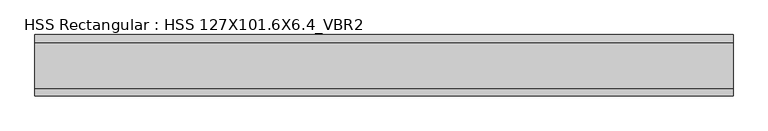
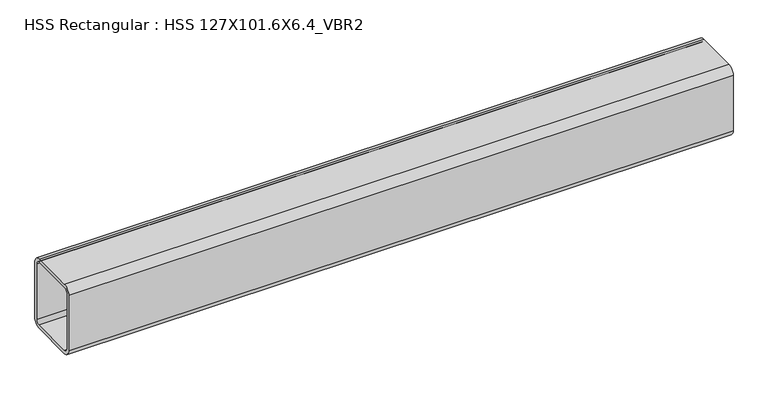
"""IFC4 building model written with IfcOpenShell, lengths in millimetres: member geometry, HSS Rectangular : HSS 127X101.6X6.4_VBR2."""

from ifc_helpers import new_model, si_unit, point, frame, frame_2d, origin, place, context, project, spatial, polyline, circle_curve, trimmed, segment, composite_curve, outline, extrude, source, transform, mapped, element, save


def hss_rectangular_hss_127x101_6x6_4_vbr2_0793e8e8(model_context):
    return source(origin(), model_context, "Body", "SweptSolid", [
        extrude(outline(composite_curve([segment(polyline([(50.8, 50.8), (50.8, -50.8)]), True, "CONTINUOUS"), segment(trimmed(circle_curve(frame_2d((38.1, -50.8)), 12.7), [point((50.8, -50.8))], [point((38.1, -63.5))], False, "CARTESIAN"), True, "CONTINUOUS"), segment(polyline([(38.1, -63.5), (-38.1, -63.5)]), True, "CONTINUOUS"), segment(trimmed(circle_curve(frame_2d((-38.1, -50.8)), 12.7), [point((-38.1, -63.5))], [point((-50.8, -50.8))], False, "CARTESIAN"), True, "CONTINUOUS"), segment(polyline([(-50.8, -50.8), (-50.8, 50.8)]), True, "CONTINUOUS"), segment(trimmed(circle_curve(frame_2d((-38.1, 50.8)), 12.7), [point((-50.8, 50.8))], [point((-38.1, 63.5))], False, "CARTESIAN"), True, "CONTINUOUS"), segment(polyline([(-38.1, 63.5), (38.1, 63.5)]), True, "CONTINUOUS"), segment(trimmed(circle_curve(frame_2d((38.1, 50.8)), 12.7), [point((38.1, 63.5))], [point((50.8, 50.8))], False, "CARTESIAN"), True, "CONTINUOUS")], self_intersect=False), holes=[composite_curve([segment(trimmed(circle_curve(frame_2d((-38.1, 50.8)), 6.35), [point((-38.1, 57.15))], [point((-44.45, 50.8))], True, "CARTESIAN"), True, "CONTINUOUS"), segment(polyline([(-44.45, 50.8), (-44.45, -50.8)]), True, "CONTINUOUS"), segment(trimmed(circle_curve(frame_2d((-38.1, -50.8)), 6.35), [point((-44.45, -50.8))], [point((-38.1, -57.15))], True, "CARTESIAN"), True, "CONTINUOUS"), segment(polyline([(-38.1, -57.15), (38.1, -57.15)]), True, "CONTINUOUS"), segment(trimmed(circle_curve(frame_2d((38.1, -50.8)), 6.35), [point((38.1, -57.15))], [point((44.45, -50.8))], True, "CARTESIAN"), True, "CONTINUOUS"), segment(polyline([(44.45, -50.8), (44.45, 50.8)]), True, "CONTINUOUS"), segment(trimmed(circle_curve(frame_2d((38.1, 50.8)), 6.35), [point((44.45, 50.8))], [point((38.1, 57.15))], True, "CARTESIAN"), True, "CONTINUOUS"), segment(polyline([(38.1, 57.15), (-38.1, 57.15)]), True, "CONTINUOUS")], self_intersect=False)]), frame((-613.1910365, 0.0, 0.0), z_axis=(1.0, 0.0, 0.0), x_axis=(0.0, 1.0, 0.0)), (0.0, 0.0, 1.0), 1153.1966521),
    ])


if __name__ == "__main__":
    model = new_model("IFC4")
    model_context = context("Model", 3, world=origin())
    ifc_project = project(units=[si_unit("LENGTHUNIT", "METRE", prefix="MILLI")], contexts=[model_context])
    site = spatial("IfcSite", under=ifc_project)
    building = spatial("IfcBuilding", under=site)
    placement = place(None, origin())
    hss_rectangular_hss_127x101_6x6_4_vbr2_shape = hss_rectangular_hss_127x101_6x6_4_vbr2_0793e8e8(model_context)
    element("IfcMember", 1, ObjectType="HSS Rectangular : HSS 127X101.6X6.4_VBR2", at=placement, inside=building, context=model_context, shape_type="MappedRepresentation", body=[
        mapped(hss_rectangular_hss_127x101_6x6_4_vbr2_shape, transform((0.0, 0.0, 0.0), x_axis=(1.0, 0.0, 0.0), y_axis=(0.0, 1.0, 0.0), z_axis=(0.0, 0.0, 1.0))),
    ])
    save(model, "model.ifc")

# Revit data of these elements
# Type "HSS Rectangular : HSS 127X101.6X6.4_VBR2"
#   Section Name Key = "HSS5X4X1/4"
#   Assembly Code = "B10"
#   Width = 10.16 cm
#   Wall Nominal Thickness = 0.635 cm
#   Wall Design Thickness = 0.5918 cm
#   Torsional Moment of Inertia = 749.217 cm⁴
#   Torsional Modulus = 136.34 cm³
#   Section Area = 24.7741 cm²
#   Plastic Modulus weak axis = 91.2759 cm³
#   Plastic Modulus strong axis = 106.352 cm³
#   Perimeter = 0.435254 m²/m
#   Outer Fillet = 1.27 cm
#   Nominal Weight = 20.7004 kgf/m
#   Moment of Inertia weak axis = 393.755 cm⁴
#   Moment of Inertia strong axis = 557.75 cm⁴
#   Inner Fillet = 0.635 cm
#   Height = 12.7 cm
#   Elastic Modulus weak axis = 77.5108 cm³
#   Elastic Modulus strong axis = 87.6708 cm³
#   Centroid Vertical = 6.35 cm
#   Centroid Horizontal = 5.08 cm
#   Length [instance default] = 1524 mm
#   Structural Material [instance default] = Steel ASTM A500, Grade C, Rectangular and Square
#   Principal Axes Angle = 0
# Element 1 (IfcMember, "HSS Rectangular : HSS 127X101.6X6.4_VBR2")
#   Materials on its faces: "Steel ASTM A500, Grade C, Rectangular and Square"
# Materials
#   "Steel ASTM A500, Grade C, Rectangular and Square": class "Metal", colour RGB 120 120 120, transparency 0, Description = "Carbon steel", Cost = 0
